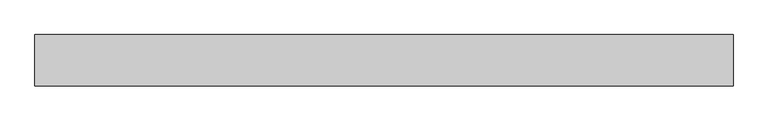
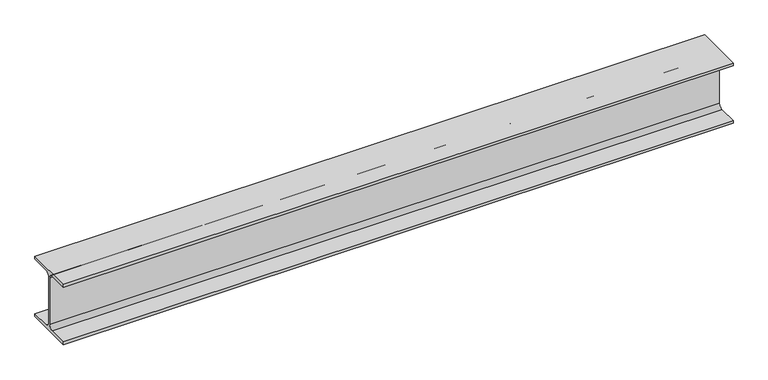
"""IFC4 building model written with IfcOpenShell, lengths in millimetres: beam geometry, 0912_Steel Framing_H-KSD3502 : H_SB_ASB_H-194x150x6x9."""

from ifc_helpers import new_model, si_unit, point, frame, frame_2d, origin, place, context, project, spatial, polyline, circle_curve, trimmed, segment, composite_curve, outline, extrude, source, transform, mapped, element, save


def beam_6c767914(model_context):
    return source(origin(), model_context, "Body", "SweptSolid", [
        extrude(outline(composite_curve([segment(polyline([(75.0, -88.0), (75.0, -97.0), (-75.0, -97.0), (-75.0, -88.0), (-16.0, -88.0)]), True, "CONTINUOUS"), segment(trimmed(circle_curve(frame_2d((-16.0, -75.0)), 13.0), [point((-16.0, -88.0))], [point((-3.0, -75.0))], True, "CARTESIAN"), True, "CONTINUOUS"), segment(polyline([(-3.0, -75.0), (-3.0, 75.0)]), True, "CONTINUOUS"), segment(trimmed(circle_curve(frame_2d((-16.0, 75.0)), 13.0), [point((-3.0, 75.0))], [point((-16.0, 88.0))], True, "CARTESIAN"), True, "CONTINUOUS"), segment(polyline([(-16.0, 88.0), (-75.0, 88.0), (-75.0, 97.0), (75.0, 97.0), (75.0, 88.0), (16.0, 88.0)]), True, "CONTINUOUS"), segment(trimmed(circle_curve(frame_2d((16.0, 75.0)), 13.0), [point((16.0, 88.0))], [point((3.0, 75.0))], True, "CARTESIAN"), True, "CONTINUOUS"), segment(polyline([(3.0, 75.0), (3.0, -75.0)]), True, "CONTINUOUS"), segment(trimmed(circle_curve(frame_2d((16.0, -75.0)), 13.0), [point((3.0, -75.0))], [point((16.0, -88.0))], True, "CARTESIAN"), True, "CONTINUOUS"), segment(polyline([(16.0, -88.0), (75.0, -88.0)]), True, "CONTINUOUS")], self_intersect=False)), frame((-1172.13, 0.0, 0.0), z_axis=(1.0, 0.0, 0.0), x_axis=(0.0, 1.0, 0.0)), (0.0, 0.0, 1.0), 2039.3467737),
    ])


if __name__ == "__main__":
    model = new_model("IFC4")
    model_context = context("Model", 3, world=origin())
    ifc_project = project(units=[si_unit("LENGTHUNIT", "METRE", prefix="MILLI")], contexts=[model_context])
    site = spatial("IfcSite", under=ifc_project)
    building = spatial("IfcBuilding", under=site)
    placement = place(None, origin())
    beam_shape = beam_6c767914(model_context)
    element("IfcBeam", 1, ObjectType="0912_Steel Framing_H-KSD3502 : H_SB_ASB_H-194x150x6x9", at=placement, inside=building, context=model_context, shape_type="MappedRepresentation", body=[
        mapped(beam_shape, transform((0.0, 0.0, 0.0), x_axis=(1.0, 0.0, 0.0), y_axis=(0.0, 1.0, 0.0), z_axis=(0.0, 0.0, 1.0))),
    ])
    save(model, "model.ifc")

# Revit data of these elements
# Type "0912_Steel Framing_H-KSD3502 : H_SB_ASB_H-194x150x6x9"
#   H_WM Code_1 = "S01AA002-00001 | Main Steel Structure Fabrication Work | Shelter/Building | Medium Steel - Standard (90KG/M>Weight≥30KG/M) | Material: (   )"
#   H_WM Code_2 = "S03AA028-00001 | Main Steel Structure Erection Work | Shelter/Building | Medium Steel (90KG/M>Weight≥30KG/M) | Material: (   )"
#   H_WM Code_3 = "S01AA010-00001 | Main Steel Structure Fabrication Work | Shelter/Building | Steel Painting/Coating | for Non-Fireproofed Steel Surface, Surface Preparation, Primer, Second & Final Coat | Material: (   )"
#   H_Q'ty Cal Type Tag = "SB-Q2"
#   Width = 15.0 cm
#   Web Thickness = 0.6 cm
#   Web Fillet = 1.3 cm
#   Warping Constant = 43316.0 cm⁶
#   W = 0
#   Torsional Moment of Inertia = 8.622 cm⁴
#   Section Area = 39.01 cm²
#   Plastic Modulus weak axis = 104.0 cm³
#   Plastic Modulus strong axis = 309.0 cm³
#   Perimeter = 0.95 m²/m
#   Nominal Weight = 30.60 kgf/m
#   Moment of Inertia weak axis = 507.00 cm⁴
#   Moment of Inertia strong axis = 2690.00 cm⁴
#   Height = 19.4 cm
#   Flange Thickness = 0.9 cm
#   Elastic Modulus weak axis = 67.6 cm³
#   Elastic Modulus strong axis = 277.0 cm³
#   Centroid Vertical = 9.7 cm
#   Centroid Horizontal = 7.5 cm
#   Ix = 26900000
#   Length [instance default] = 1.5240 m
#   Zx = 309000
#   b = 0.1500 m
#   h = 0.1940 m
#   r = 0.0130 m
#   s = 0.0060 m
#   t = 0.0090 m
#   A = 0.003901 m²
#   Structural Material [instance default] = Steel, 45-345
#   Assembly Code = ""
# Element 1 (IfcBeam, "0912_Steel Framing_H-KSD3502 : H_SB_ASB_H-194x150x6x9")
#   Structural Material = none
# Materials
#   "Steel, 45-345": class "Metal", colour RGB 189 187 185, transparency 0, Description = "Steel 345 MPa", Cost = 0
